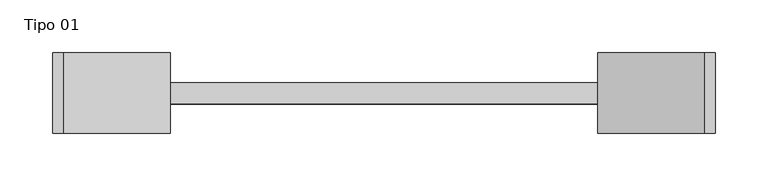
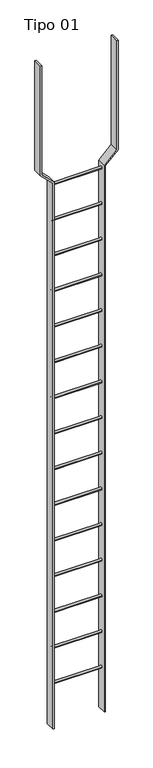
"""IFC4 building model written with IfcOpenShell, lengths in millimetres: proxy geometry, Escada Marinheiro : Tipo 01."""

from ifc_helpers import new_model, si_unit, point, frame, frame_2d, origin, place, context, project, spatial, polyline, circle_curve, trimmed, segment, composite_curve, outline, extrude, source, transform, mapped, element, save


def tipo_01_c6b6edbc(model_context):
    return source(origin(), model_context, "Body", "SweptSolid", [
        extrude(outline(composite_curve([segment(trimmed(circle_curve(frame_2d((286.0, -4270.0)), 10.0), [point((276.0, -4270.0))], [point((296.0, -4270.0))], False, "CARTESIAN"), True, "CONTINUOUS"), segment(trimmed(circle_curve(frame_2d((286.0, -4270.0)), 10.0), [point((296.0, -4270.0))], [point((276.0, -4270.0))], False, "CARTESIAN"), True, "CONTINUOUS")], self_intersect=False)), frame((-202.5, 0.0, 0.0), z_axis=(1.0, 0.0, 0.0), x_axis=(0.0, 1.0, 0.0)), (0.0, 0.0, 1.0), 405.0),
        extrude(outline(composite_curve([segment(trimmed(circle_curve(frame_2d((286.0, -3965.0)), 10.0), [point((276.0, -3965.0))], [point((296.0, -3965.0))], False, "CARTESIAN"), True, "CONTINUOUS"), segment(trimmed(circle_curve(frame_2d((286.0, -3965.0)), 10.0), [point((296.0, -3965.0))], [point((276.0, -3965.0))], False, "CARTESIAN"), True, "CONTINUOUS")], self_intersect=False)), frame((-202.5, 0.0, 0.0), z_axis=(1.0, 0.0, 0.0), x_axis=(0.0, 1.0, 0.0)), (0.0, 0.0, 1.0), 405.0),
        extrude(outline(composite_curve([segment(trimmed(circle_curve(frame_2d((286.0, -3660.0)), 10.0), [point((276.0, -3660.0))], [point((296.0, -3660.0))], False, "CARTESIAN"), True, "CONTINUOUS"), segment(trimmed(circle_curve(frame_2d((286.0, -3660.0)), 10.0), [point((296.0, -3660.0))], [point((276.0, -3660.0))], False, "CARTESIAN"), True, "CONTINUOUS")], self_intersect=False)), frame((-202.5, 0.0, 0.0), z_axis=(1.0, 0.0, 0.0), x_axis=(0.0, 1.0, 0.0)), (0.0, 0.0, 1.0), 405.0),
        extrude(outline(composite_curve([segment(trimmed(circle_curve(frame_2d((286.0, -3355.0)), 10.0), [point((276.0, -3355.0))], [point((296.0, -3355.0))], False, "CARTESIAN"), True, "CONTINUOUS"), segment(trimmed(circle_curve(frame_2d((286.0, -3355.0)), 10.0), [point((296.0, -3355.0))], [point((276.0, -3355.0))], False, "CARTESIAN"), True, "CONTINUOUS")], self_intersect=False)), frame((-202.5, 0.0, 0.0), z_axis=(1.0, 0.0, 0.0), x_axis=(0.0, 1.0, 0.0)), (0.0, 0.0, 1.0), 405.0),
        extrude(outline(composite_curve([segment(trimmed(circle_curve(frame_2d((286.0, -3050.0)), 10.0), [point((276.0, -3050.0))], [point((296.0, -3050.0))], False, "CARTESIAN"), True, "CONTINUOUS"), segment(trimmed(circle_curve(frame_2d((286.0, -3050.0)), 10.0), [point((296.0, -3050.0))], [point((276.0, -3050.0))], False, "CARTESIAN"), True, "CONTINUOUS")], self_intersect=False)), frame((-202.5, 0.0, 0.0), z_axis=(1.0, 0.0, 0.0), x_axis=(0.0, 1.0, 0.0)), (0.0, 0.0, 1.0), 405.0),
        extrude(outline(composite_curve([segment(trimmed(circle_curve(frame_2d((286.0, -2745.0)), 10.0), [point((276.0, -2745.0))], [point((296.0, -2745.0))], False, "CARTESIAN"), True, "CONTINUOUS"), segment(trimmed(circle_curve(frame_2d((286.0, -2745.0)), 10.0), [point((296.0, -2745.0))], [point((276.0, -2745.0))], False, "CARTESIAN"), True, "CONTINUOUS")], self_intersect=False)), frame((-202.5, 0.0, 0.0), z_axis=(1.0, 0.0, 0.0), x_axis=(0.0, 1.0, 0.0)), (0.0, 0.0, 1.0), 405.0),
        extrude(outline(composite_curve([segment(trimmed(circle_curve(frame_2d((286.0, -2440.0)), 10.0), [point((276.0, -2440.0))], [point((296.0, -2440.0))], False, "CARTESIAN"), True, "CONTINUOUS"), segment(trimmed(circle_curve(frame_2d((286.0, -2440.0)), 10.0), [point((296.0, -2440.0))], [point((276.0, -2440.0))], False, "CARTESIAN"), True, "CONTINUOUS")], self_intersect=False)), frame((-202.5, 0.0, 0.0), z_axis=(1.0, 0.0, 0.0), x_axis=(0.0, 1.0, 0.0)), (0.0, 0.0, 1.0), 405.0),
        extrude(outline(composite_curve([segment(trimmed(circle_curve(frame_2d((286.0, -2135.0)), 10.0), [point((276.0, -2135.0))], [point((296.0, -2135.0))], False, "CARTESIAN"), True, "CONTINUOUS"), segment(trimmed(circle_curve(frame_2d((286.0, -2135.0)), 10.0), [point((296.0, -2135.0))], [point((276.0, -2135.0))], False, "CARTESIAN"), True, "CONTINUOUS")], self_intersect=False)), frame((-202.5, 0.0, 0.0), z_axis=(1.0, 0.0, 0.0), x_axis=(0.0, 1.0, 0.0)), (0.0, 0.0, 1.0), 405.0),
        extrude(outline(composite_curve([segment(trimmed(circle_curve(frame_2d((286.0, -1830.0)), 10.0), [point((276.0, -1830.0))], [point((296.0, -1830.0))], False, "CARTESIAN"), True, "CONTINUOUS"), segment(trimmed(circle_curve(frame_2d((286.0, -1830.0)), 10.0), [point((296.0, -1830.0))], [point((276.0, -1830.0))], False, "CARTESIAN"), True, "CONTINUOUS")], self_intersect=False)), frame((-202.5, 0.0, 0.0), z_axis=(1.0, 0.0, 0.0), x_axis=(0.0, 1.0, 0.0)), (0.0, 0.0, 1.0), 405.0),
        extrude(outline(composite_curve([segment(trimmed(circle_curve(frame_2d((286.0, -1525.0)), 10.0), [point((276.0, -1525.0))], [point((296.0, -1525.0))], False, "CARTESIAN"), True, "CONTINUOUS"), segment(trimmed(circle_curve(frame_2d((286.0, -1525.0)), 10.0), [point((296.0, -1525.0))], [point((276.0, -1525.0))], False, "CARTESIAN"), True, "CONTINUOUS")], self_intersect=False)), frame((-202.5, 0.0, 0.0), z_axis=(1.0, 0.0, 0.0), x_axis=(0.0, 1.0, 0.0)), (0.0, 0.0, 1.0), 405.0),
        extrude(outline(composite_curve([segment(trimmed(circle_curve(frame_2d((286.0, -1220.0)), 10.0), [point((276.0, -1220.0))], [point((296.0, -1220.0))], False, "CARTESIAN"), True, "CONTINUOUS"), segment(trimmed(circle_curve(frame_2d((286.0, -1220.0)), 10.0), [point((296.0, -1220.0))], [point((276.0, -1220.0))], False, "CARTESIAN"), True, "CONTINUOUS")], self_intersect=False)), frame((-202.5, 0.0, 0.0), z_axis=(1.0, 0.0, 0.0), x_axis=(0.0, 1.0, 0.0)), (0.0, 0.0, 1.0), 405.0),
        extrude(outline(composite_curve([segment(trimmed(circle_curve(frame_2d((286.0, -915.0)), 10.0), [point((276.0, -915.0))], [point((296.0, -915.0))], False, "CARTESIAN"), True, "CONTINUOUS"), segment(trimmed(circle_curve(frame_2d((286.0, -915.0)), 10.0), [point((296.0, -915.0))], [point((276.0, -915.0))], False, "CARTESIAN"), True, "CONTINUOUS")], self_intersect=False)), frame((-202.5, 0.0, 0.0), z_axis=(1.0, 0.0, 0.0), x_axis=(0.0, 1.0, 0.0)), (0.0, 0.0, 1.0), 405.0),
        extrude(outline(composite_curve([segment(trimmed(circle_curve(frame_2d((286.0, -610.0)), 10.0), [point((276.0, -610.0))], [point((296.0, -610.0))], False, "CARTESIAN"), True, "CONTINUOUS"), segment(trimmed(circle_curve(frame_2d((286.0, -610.0)), 10.0), [point((296.0, -610.0))], [point((276.0, -610.0))], False, "CARTESIAN"), True, "CONTINUOUS")], self_intersect=False)), frame((-202.5, 0.0, 0.0), z_axis=(1.0, 0.0, 0.0), x_axis=(0.0, 1.0, 0.0)), (0.0, 0.0, 1.0), 405.0),
        extrude(outline(composite_curve([segment(trimmed(circle_curve(frame_2d((286.0, -305.0)), 10.0), [point((276.0, -305.0))], [point((296.0, -305.0))], False, "CARTESIAN"), True, "CONTINUOUS"), segment(trimmed(circle_curve(frame_2d((286.0, -305.0)), 10.0), [point((296.0, -305.0))], [point((276.0, -305.0))], False, "CARTESIAN"), True, "CONTINUOUS")], self_intersect=False)), frame((-202.5, 0.0, 0.0), z_axis=(1.0, 0.0, 0.0), x_axis=(0.0, 1.0, 0.0)), (0.0, 0.0, 1.0), 405.0),
        extrude(outline(composite_curve([segment(trimmed(circle_curve(frame_2d((286.0, 0.0)), 10.0), [point((276.0, 0.0))], [point((296.0, 0.0))], False, "CARTESIAN"), True, "CONTINUOUS"), segment(trimmed(circle_curve(frame_2d((286.0, 0.0)), 10.0), [point((296.0, 0.0))], [point((276.0, 0.0))], False, "CARTESIAN"), True, "CONTINUOUS")], self_intersect=False)), frame((-202.5, 0.0, 0.0), z_axis=(1.0, 0.0, 0.0), x_axis=(0.0, 1.0, 0.0)), (0.0, 0.0, 1.0), 405.0),
        extrude(outline(polyline([(1070.0, -314.1), (133.35, -314.1), (31.75, -212.5), (-4635.0, -212.5), (-4635.0, -202.5), (35.8921356, -202.5), (137.4921356, -304.1), (1070.0, -304.1), (1070.0, -314.1)])), frame((0.0, 247.9, 0.0), z_axis=(0.0, 1.0, 0.0), x_axis=(0.0, 0.0, 1.0)), (0.0, 0.0, 1.0), 76.2),
        extrude(outline(polyline([(1070.0, 304.1), (137.4921356, 304.1), (35.8921356, 202.5), (-4635.0, 202.5), (-4635.0, 212.5), (31.75, 212.5), (133.35, 314.1), (1070.0, 314.1), (1070.0, 304.1)])), frame((0.0, 247.9, 0.0), z_axis=(0.0, 1.0, 0.0), x_axis=(0.0, 0.0, 1.0)), (0.0, 0.0, 1.0), 76.2),
    ])


if __name__ == "__main__":
    model = new_model("IFC4")
    model_context = context("Model", 3, world=origin())
    ifc_project = project(units=[si_unit("LENGTHUNIT", "METRE", prefix="MILLI")], contexts=[model_context])
    site = spatial("IfcSite", under=ifc_project)
    building = spatial("IfcBuilding", under=site)
    placement = place(None, origin())
    tipo_01_shape = tipo_01_c6b6edbc(model_context)
    element("IfcBuildingElementProxy", 1, Name="Escada Marinheiro : Tipo 01", ObjectType="Escada Marinheiro : Tipo 01", at=placement, inside=building, context=model_context, shape_type="MappedRepresentation", body=[
        mapped(tipo_01_shape, transform((0.0, 0.0, 0.0), x_axis=(1.0, 0.0, 0.0), y_axis=(0.0, 1.0, 0.0), z_axis=(0.0, 0.0, 1.0))),
    ])
    save(model, "model.ifc")

# Revit data of these elements
# Type "Escada Marinheiro : Tipo 01"
#   Raio Barra = 1.00 cm
#   Comprimento Barra [instance default] = 40.50 cm
#   Espessura Apoio Lateral = 7.62 cm
#   Profundidade Apoio Lateral = 1.00 cm
#   Altura Base Guarda-Corpo = 53.50 cm
#   Altura [instance default] = 463.50 cm
#   Comprimento Guarda-Corpo = 51.00 cm
#   Altura Guarda-Corpo = 107.00 cm
#   Distância [instance default] = 18.00 cm
#   Espaço entre barras [instance default] = 30.50 cm
#   Number of Rungs [instance default] = 15
#   Assembly Code = ""
